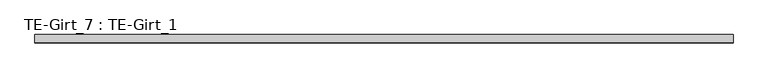
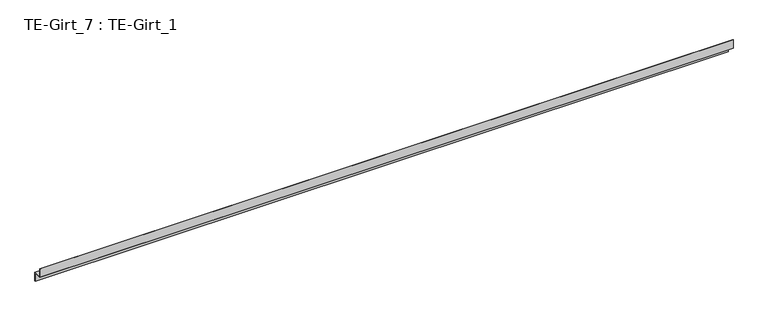
"""IFC4 building model written with IfcOpenShell, lengths in millimetres: proxy geometry, TE-Girt_7 : TE-Girt_1."""

import ifcopenshell
import ifcopenshell.guid

model = None  # the IFC model being written
_history = None  # IfcOwnerHistory: only IFC2X3 demands one
_inside = {}  # id of a spatial element -> (the spatial element, [elements in it])
_under = {}  # id of a project, library or spatial element -> (it, [spatial elements below it])
_declared = {}  # id of a project -> (the project, [libraries it declares])
_typed = {}  # id of a type object -> (the type object, [elements of that type])
_made_of = {}  # id of a material, layer set ... -> (it, [elements and type objects made of it])


def new_model(schema):
    """Start an empty IFC model of exactly this schema.

    Asked for "IFC4X3", IfcOpenShell would pick the latest addendum, in which some entities
    have other attributes; the version numbers below select the first issue.
    IFC2X3 requires an IfcOwnerHistory on every rooted entity: one is made here for all.
    """
    global model, _history
    if schema == "IFC4X3":
        model = ifcopenshell.file(schema_version=(4, 3, 0, 0))
    else:
        model = ifcopenshell.file(schema=schema)
    _inside.clear()
    _under.clear()
    _declared.clear()
    _typed.clear()
    _made_of.clear()
    _history = None
    if model.schema == "IFC2X3":
        org = make("IfcOrganization", Name="unknown")
        user = make(
            "IfcPersonAndOrganization",
            ThePerson=make("IfcPerson", FamilyName="unknown"),
            TheOrganization=org,
        )
        app = make(
            "IfcApplication",
            ApplicationDeveloper=org,
            Version="unknown",
            ApplicationFullName="unknown",
            ApplicationIdentifier="unknown",
        )
        _history = make(
            "IfcOwnerHistory",
            OwningUser=user,
            OwningApplication=app,
            ChangeAction="ADDED",
            CreationDate=0,
        )
    return model


def make(cls, **values):
    """One entity of the class cls with the attributes given. An attribute that is None is left unset."""
    return model.create_entity(
        cls, **{name: value for name, value in values.items() if value is not None}
    )


def rooted(cls, **values):
    """An entity with a GlobalId (a new one), such as an element, a storey or a relation."""
    return make(cls, GlobalId=ifcopenshell.guid.new(), OwnerHistory=_history, **values)


def si_unit(unit_type, name, prefix=None):
    """IfcSIUnit, for example si_unit("LENGTHUNIT", "METRE", prefix="MILLI")."""
    return make("IfcSIUnit", UnitType=unit_type, Prefix=prefix, Name=name)


def assignment(units):
    """IfcUnitAssignment: the units of a project."""
    return None if units is None else make("IfcUnitAssignment", Units=units)


def point(xyz):
    """IfcCartesianPoint."""
    return None if xyz is None else make("IfcCartesianPoint", Coordinates=xyz)


def direction(xyz):
    """IfcDirection."""
    return None if xyz is None else make("IfcDirection", DirectionRatios=xyz)


def frame(location, z_axis=None, x_axis=None):
    """IfcAxis2Placement3D, a coordinate frame: its origin and axes. An axis left out is left unset."""
    return make(
        "IfcAxis2Placement3D",
        Location=point(location),
        Axis=direction(z_axis),
        RefDirection=direction(x_axis),
    )


def origin():
    """The frame at (0, 0, 0) with its axes left unset."""
    return frame((0.0, 0.0, 0.0))


def place(relative_to, where):
    """IfcLocalPlacement: puts the frame where relative to a parent placement (None: the world)."""
    return make(
        "IfcLocalPlacement", PlacementRelTo=relative_to, RelativePlacement=where
    )


def context(
    kind, dimensions, precision=None, world=None, true_north=None, identifier=None
):
    """IfcGeometricRepresentationContext, for example the 3D "Model" context."""
    return make(
        "IfcGeometricRepresentationContext",
        ContextIdentifier=identifier,
        ContextType=kind,
        CoordinateSpaceDimension=dimensions,
        Precision=precision,
        WorldCoordinateSystem=world,
        TrueNorth=true_north,
    )


def project(units=None, contexts=None):
    """IfcProject with its units and contexts."""
    return rooted(
        "IfcProject",
        Name="project",
        RepresentationContexts=contexts,
        UnitsInContext=assignment(units),
    )


def spatial(cls, under=None, at=None, **own):
    """A site, building, storey or space (cls), placed at a placement, below another one or the project."""
    s = rooted(cls, ObjectPlacement=at, **own)
    if under is not None:
        _under.setdefault(under.id(), (under, []))[1].append(s)
    return s


def polyline(points):
    """IfcPolyline through the points."""
    return make("IfcPolyline", Points=[point(p) for p in points])


def outline(outer, holes=None, kind="AREA"):
    """IfcArbitraryClosedProfileDef: a profile drawn as a closed curve; with holes, ...WithVoids."""
    if holes is None:
        return make("IfcArbitraryClosedProfileDef", ProfileType=kind, OuterCurve=outer)
    return make(
        "IfcArbitraryProfileDefWithVoids",
        ProfileType=kind,
        OuterCurve=outer,
        InnerCurves=holes,
    )


def extrude(swept, where, along, depth):
    """IfcExtrudedAreaSolid: the profile swept, set in the frame where, extruded along a direction by depth."""
    return make(
        "IfcExtrudedAreaSolid",
        SweptArea=swept,
        Position=where,
        ExtrudedDirection=direction(along),
        Depth=depth,
    )


def shape(context_of_items, identifier, shape_type, items):
    """IfcShapeRepresentation: the items that make up one representation, for example the "Body"."""
    return make(
        "IfcShapeRepresentation",
        ContextOfItems=context_of_items,
        RepresentationIdentifier=identifier,
        RepresentationType=shape_type,
        Items=items,
    )


def source(mapping_origin, context_of_items, identifier, shape_type, items):
    """IfcRepresentationMap: a shape defined once, which mapped items show again and again."""
    return make(
        "IfcRepresentationMap",
        MappingOrigin=mapping_origin,
        MappedRepresentation=shape(context_of_items, identifier, shape_type, items),
    )


def transform(
    local_origin,
    x_axis=None,
    y_axis=None,
    z_axis=None,
    scale=None,
    scale2=None,
    scale3=None,
    uniform=True,
):
    """IfcCartesianTransformationOperator3D, or its non-uniform kind. x_axis, y_axis, z_axis: its Axis1, 2, 3."""
    if uniform:
        return make(
            "IfcCartesianTransformationOperator3D",
            Axis1=direction(x_axis),
            Axis2=direction(y_axis),
            LocalOrigin=point(local_origin),
            Scale=scale,
            Axis3=direction(z_axis),
        )
    return make(
        "IfcCartesianTransformationOperator3DnonUniform",
        Axis1=direction(x_axis),
        Axis2=direction(y_axis),
        LocalOrigin=point(local_origin),
        Scale=scale,
        Axis3=direction(z_axis),
        Scale2=scale2,
        Scale3=scale3,
    )


def mapped(mapping_source, mapping_target):
    """IfcMappedItem: shows the shape of a source again, moved by a transform."""
    return make(
        "IfcMappedItem", MappingSource=mapping_source, MappingTarget=mapping_target
    )


def made_of(thing, what):
    """Note that an element or type object is made of a material, layer set ...; save() writes the relation."""
    if what is not None:
        _made_of.setdefault(what.id(), (what, []))[1].append(thing)
    return thing


def element(
    cls,
    number,
    at=None,
    inside=None,
    cuts=None,
    type_object=None,
    material=None,
    context=None,
    identifier="Body",
    shape_type=None,
    held_by="IfcProductDefinitionShape",
    body=None,
    shapes=None,
    **own,
):
    """One element of the class cls, such as IfcWall. Its Tag is "e" and its number.

    at: its placement. inside: the storey or other place that contains it. cuts: it is an
    opening in that element (IfcRelVoidsElement). A single representation is given by context,
    identifier, shape_type and body (its items); several are given by shapes. held_by: the class
    of the entity that holds the representations. save() writes the other relations.
    """
    e = rooted(cls, Tag="e%d" % number, ObjectPlacement=at, **own)
    if body is not None:
        shapes = [shape(context, identifier, shape_type, body)]
    if shapes is not None:
        e.Representation = make(held_by, Representations=shapes)
    if inside is not None:
        _inside.setdefault(inside.id(), (inside, []))[1].append(e)
    if cuts is not None:
        rooted(
            "IfcRelVoidsElement", RelatingBuildingElement=cuts, RelatedOpeningElement=e
        )
    if type_object is not None:
        _typed.setdefault(type_object.id(), (type_object, []))[1].append(e)
    return made_of(e, material)


def aggregate(whole, parts):
    """IfcRelAggregates: a whole, such as a stair, and the parts it consists of."""
    return rooted("IfcRelAggregates", RelatingObject=whole, RelatedObjects=parts)


def save(model, path):
    """Write the relations noted so far, then the file.

    IfcRelAggregates (storeys below a building ...), IfcRelContainedInSpatialStructure (elements
    in a storey), IfcRelDefinesByType, IfcRelAssociatesMaterial and IfcRelDeclares: one each for
    every whole, place, type object, material and project.
    """
    for whole, parts in _under.values():
        aggregate(whole, parts)
    for where, things in _inside.values():
        rooted(
            "IfcRelContainedInSpatialStructure",
            RelatedElements=things,
            RelatingStructure=where,
        )
    for kind, things in _typed.values():
        rooted("IfcRelDefinesByType", RelatedObjects=things, RelatingType=kind)
    for what, things in _made_of.values():
        rooted("IfcRelAssociatesMaterial", RelatedObjects=things, RelatingMaterial=what)
    for by, libraries in _declared.values():
        rooted("IfcRelDeclares", RelatingContext=by, RelatedDefinitions=libraries)
    model.write(path)


def te_girt_7_te_girt_1_0389d321(model_context):
    return source(origin(), model_context, "Body", "SweptSolid", [
        extrude(outline(polyline([(-531639.2163841, 844.55), (-531639.2163841, 806.45), (-531640.1093528, 806.45), (-531640.1093528, 843.6570312), (-531674.1249348, 843.6570312), (-531674.1249348, 881.7570312), (-531673.231966, 881.7570312), (-531673.231966, 844.55), (-531639.2163841, 844.55)])), frame((587397.6434739, 0.0, 0.0), z_axis=(1.0, 0.0, 0.0), x_axis=(0.0, 1.0, 0.0)), (0.0, 0.0, 1.0), 2921.0),
    ])


if __name__ == "__main__":
    model = new_model("IFC4")
    model_context = context("Model", 3, world=origin())
    ifc_project = project(units=[si_unit("LENGTHUNIT", "METRE", prefix="MILLI")], contexts=[model_context])
    site = spatial("IfcSite", under=ifc_project)
    building = spatial("IfcBuilding", under=site)
    placement = place(None, origin())
    te_girt_7_te_girt_1_shape = te_girt_7_te_girt_1_0389d321(model_context)
    element("IfcBuildingElementProxy", 1, Name="TE-Girt_7 : TE-Girt_1", ObjectType="TE-Girt_7 : TE-Girt_1", at=placement, inside=building, context=model_context, shape_type="MappedRepresentation", body=[
        mapped(te_girt_7_te_girt_1_shape, transform((0.0, 0.0, 0.0), x_axis=(1.0, 0.0, 0.0), y_axis=(0.0, 1.0, 0.0), z_axis=(0.0, 0.0, 1.0))),
    ])
    save(model, "model.ifc")

# Revit data of these elements
# Element 1 (IfcBuildingElementProxy, "TE-Girt_7 : TE-Girt_1")
#   Materials on its faces: "Z-FURRING, COLD-FORMED GALV."
# Materials
#   "Z-FURRING, COLD-FORMED GALV.": class "Generic", colour RGB 143 142 141, transparency 0, Cost = 0
